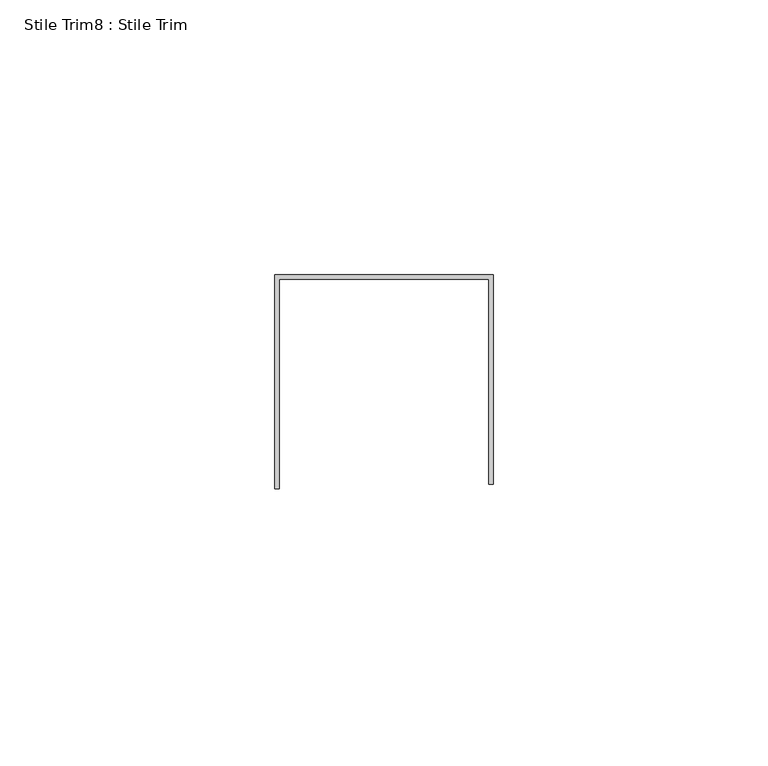
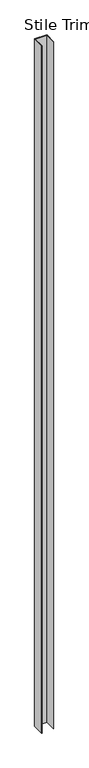
"""IFC4 building model written with IfcOpenShell, lengths in millimetres: proxy geometry, Stile Trim8 : Stile Trim."""

import ifcopenshell
import ifcopenshell.guid

model = None  # the IFC model being written
_history = None  # IfcOwnerHistory: only IFC2X3 demands one
_inside = {}  # id of a spatial element -> (the spatial element, [elements in it])
_under = {}  # id of a project, library or spatial element -> (it, [spatial elements below it])
_declared = {}  # id of a project -> (the project, [libraries it declares])
_typed = {}  # id of a type object -> (the type object, [elements of that type])
_made_of = {}  # id of a material, layer set ... -> (it, [elements and type objects made of it])


def new_model(schema):
    """Start an empty IFC model of exactly this schema.

    Asked for "IFC4X3", IfcOpenShell would pick the latest addendum, in which some entities
    have other attributes; the version numbers below select the first issue.
    IFC2X3 requires an IfcOwnerHistory on every rooted entity: one is made here for all.
    """
    global model, _history
    if schema == "IFC4X3":
        model = ifcopenshell.file(schema_version=(4, 3, 0, 0))
    else:
        model = ifcopenshell.file(schema=schema)
    _inside.clear()
    _under.clear()
    _declared.clear()
    _typed.clear()
    _made_of.clear()
    _history = None
    if model.schema == "IFC2X3":
        org = make("IfcOrganization", Name="unknown")
        user = make(
            "IfcPersonAndOrganization",
            ThePerson=make("IfcPerson", FamilyName="unknown"),
            TheOrganization=org,
        )
        app = make(
            "IfcApplication",
            ApplicationDeveloper=org,
            Version="unknown",
            ApplicationFullName="unknown",
            ApplicationIdentifier="unknown",
        )
        _history = make(
            "IfcOwnerHistory",
            OwningUser=user,
            OwningApplication=app,
            ChangeAction="ADDED",
            CreationDate=0,
        )
    return model


def make(cls, **values):
    """One entity of the class cls with the attributes given. An attribute that is None is left unset."""
    return model.create_entity(
        cls, **{name: value for name, value in values.items() if value is not None}
    )


def rooted(cls, **values):
    """An entity with a GlobalId (a new one), such as an element, a storey or a relation."""
    return make(cls, GlobalId=ifcopenshell.guid.new(), OwnerHistory=_history, **values)


def si_unit(unit_type, name, prefix=None):
    """IfcSIUnit, for example si_unit("LENGTHUNIT", "METRE", prefix="MILLI")."""
    return make("IfcSIUnit", UnitType=unit_type, Prefix=prefix, Name=name)


def assignment(units):
    """IfcUnitAssignment: the units of a project."""
    return None if units is None else make("IfcUnitAssignment", Units=units)


def point(xyz):
    """IfcCartesianPoint."""
    return None if xyz is None else make("IfcCartesianPoint", Coordinates=xyz)


def direction(xyz):
    """IfcDirection."""
    return None if xyz is None else make("IfcDirection", DirectionRatios=xyz)


def frame(location, z_axis=None, x_axis=None):
    """IfcAxis2Placement3D, a coordinate frame: its origin and axes. An axis left out is left unset."""
    return make(
        "IfcAxis2Placement3D",
        Location=point(location),
        Axis=direction(z_axis),
        RefDirection=direction(x_axis),
    )


def origin():
    """The frame at (0, 0, 0) with its axes left unset."""
    return frame((0.0, 0.0, 0.0))


def place(relative_to, where):
    """IfcLocalPlacement: puts the frame where relative to a parent placement (None: the world)."""
    return make(
        "IfcLocalPlacement", PlacementRelTo=relative_to, RelativePlacement=where
    )


def context(
    kind, dimensions, precision=None, world=None, true_north=None, identifier=None
):
    """IfcGeometricRepresentationContext, for example the 3D "Model" context."""
    return make(
        "IfcGeometricRepresentationContext",
        ContextIdentifier=identifier,
        ContextType=kind,
        CoordinateSpaceDimension=dimensions,
        Precision=precision,
        WorldCoordinateSystem=world,
        TrueNorth=true_north,
    )


def project(units=None, contexts=None):
    """IfcProject with its units and contexts."""
    return rooted(
        "IfcProject",
        Name="project",
        RepresentationContexts=contexts,
        UnitsInContext=assignment(units),
    )


def spatial(cls, under=None, at=None, **own):
    """A site, building, storey or space (cls), placed at a placement, below another one or the project."""
    s = rooted(cls, ObjectPlacement=at, **own)
    if under is not None:
        _under.setdefault(under.id(), (under, []))[1].append(s)
    return s


def polyline(points):
    """IfcPolyline through the points."""
    return make("IfcPolyline", Points=[point(p) for p in points])


def outline(outer, holes=None, kind="AREA"):
    """IfcArbitraryClosedProfileDef: a profile drawn as a closed curve; with holes, ...WithVoids."""
    if holes is None:
        return make("IfcArbitraryClosedProfileDef", ProfileType=kind, OuterCurve=outer)
    return make(
        "IfcArbitraryProfileDefWithVoids",
        ProfileType=kind,
        OuterCurve=outer,
        InnerCurves=holes,
    )


def extrude(swept, where, along, depth):
    """IfcExtrudedAreaSolid: the profile swept, set in the frame where, extruded along a direction by depth."""
    return make(
        "IfcExtrudedAreaSolid",
        SweptArea=swept,
        Position=where,
        ExtrudedDirection=direction(along),
        Depth=depth,
    )


def shape(context_of_items, identifier, shape_type, items):
    """IfcShapeRepresentation: the items that make up one representation, for example the "Body"."""
    return make(
        "IfcShapeRepresentation",
        ContextOfItems=context_of_items,
        RepresentationIdentifier=identifier,
        RepresentationType=shape_type,
        Items=items,
    )


def source(mapping_origin, context_of_items, identifier, shape_type, items):
    """IfcRepresentationMap: a shape defined once, which mapped items show again and again."""
    return make(
        "IfcRepresentationMap",
        MappingOrigin=mapping_origin,
        MappedRepresentation=shape(context_of_items, identifier, shape_type, items),
    )


def transform(
    local_origin,
    x_axis=None,
    y_axis=None,
    z_axis=None,
    scale=None,
    scale2=None,
    scale3=None,
    uniform=True,
):
    """IfcCartesianTransformationOperator3D, or its non-uniform kind. x_axis, y_axis, z_axis: its Axis1, 2, 3."""
    if uniform:
        return make(
            "IfcCartesianTransformationOperator3D",
            Axis1=direction(x_axis),
            Axis2=direction(y_axis),
            LocalOrigin=point(local_origin),
            Scale=scale,
            Axis3=direction(z_axis),
        )
    return make(
        "IfcCartesianTransformationOperator3DnonUniform",
        Axis1=direction(x_axis),
        Axis2=direction(y_axis),
        LocalOrigin=point(local_origin),
        Scale=scale,
        Axis3=direction(z_axis),
        Scale2=scale2,
        Scale3=scale3,
    )


def mapped(mapping_source, mapping_target):
    """IfcMappedItem: shows the shape of a source again, moved by a transform."""
    return make(
        "IfcMappedItem", MappingSource=mapping_source, MappingTarget=mapping_target
    )


def made_of(thing, what):
    """Note that an element or type object is made of a material, layer set ...; save() writes the relation."""
    if what is not None:
        _made_of.setdefault(what.id(), (what, []))[1].append(thing)
    return thing


def element(
    cls,
    number,
    at=None,
    inside=None,
    cuts=None,
    type_object=None,
    material=None,
    context=None,
    identifier="Body",
    shape_type=None,
    held_by="IfcProductDefinitionShape",
    body=None,
    shapes=None,
    **own,
):
    """One element of the class cls, such as IfcWall. Its Tag is "e" and its number.

    at: its placement. inside: the storey or other place that contains it. cuts: it is an
    opening in that element (IfcRelVoidsElement). A single representation is given by context,
    identifier, shape_type and body (its items); several are given by shapes. held_by: the class
    of the entity that holds the representations. save() writes the other relations.
    """
    e = rooted(cls, Tag="e%d" % number, ObjectPlacement=at, **own)
    if body is not None:
        shapes = [shape(context, identifier, shape_type, body)]
    if shapes is not None:
        e.Representation = make(held_by, Representations=shapes)
    if inside is not None:
        _inside.setdefault(inside.id(), (inside, []))[1].append(e)
    if cuts is not None:
        rooted(
            "IfcRelVoidsElement", RelatingBuildingElement=cuts, RelatedOpeningElement=e
        )
    if type_object is not None:
        _typed.setdefault(type_object.id(), (type_object, []))[1].append(e)
    return made_of(e, material)


def aggregate(whole, parts):
    """IfcRelAggregates: a whole, such as a stair, and the parts it consists of."""
    return rooted("IfcRelAggregates", RelatingObject=whole, RelatedObjects=parts)


def save(model, path):
    """Write the relations noted so far, then the file.

    IfcRelAggregates (storeys below a building ...), IfcRelContainedInSpatialStructure (elements
    in a storey), IfcRelDefinesByType, IfcRelAssociatesMaterial and IfcRelDeclares: one each for
    every whole, place, type object, material and project.
    """
    for whole, parts in _under.values():
        aggregate(whole, parts)
    for where, things in _inside.values():
        rooted(
            "IfcRelContainedInSpatialStructure",
            RelatedElements=things,
            RelatingStructure=where,
        )
    for kind, things in _typed.values():
        rooted("IfcRelDefinesByType", RelatedObjects=things, RelatingType=kind)
    for what, things in _made_of.values():
        rooted("IfcRelAssociatesMaterial", RelatedObjects=things, RelatingMaterial=what)
    for by, libraries in _declared.values():
        rooted("IfcRelDeclares", RelatingContext=by, RelatedDefinitions=libraries)
    model.write(path)


def stile_trim8_stile_trim_18cce888(model_context):
    return source(origin(), model_context, "Body", "SweptSolid", [
        extrude(outline(polyline([(587327.0060739, -535207.1289841), (587366.6808739, -535207.1289841), (587366.6808739, -535245.2289841), (587365.8934739, -535245.2289841), (587365.8934739, -535207.9163841), (587327.7934739, -535207.9163841), (587327.7934739, -535246.0163841), (587327.0060739, -535246.0163841), (587327.0060739, -535207.1289841)])), frame((0.0, 0.0, 50.8), z_axis=(0.0, 0.0, 1.0), x_axis=(1.0, 0.0, 0.0)), (0.0, 0.0, 1.0), 2350.3929688),
    ])


if __name__ == "__main__":
    model = new_model("IFC4")
    model_context = context("Model", 3, world=origin())
    ifc_project = project(units=[si_unit("LENGTHUNIT", "METRE", prefix="MILLI")], contexts=[model_context])
    site = spatial("IfcSite", under=ifc_project)
    building = spatial("IfcBuilding", under=site)
    placement = place(None, origin())
    stile_trim8_stile_trim_shape = stile_trim8_stile_trim_18cce888(model_context)
    element("IfcBuildingElementProxy", 1, Name="Stile Trim8 : Stile Trim", ObjectType="Stile Trim8 : Stile Trim", at=placement, inside=building, context=model_context, shape_type="MappedRepresentation", body=[
        mapped(stile_trim8_stile_trim_shape, transform((0.0, 0.0, 0.0), x_axis=(1.0, 0.0, 0.0), y_axis=(0.0, 1.0, 0.0), z_axis=(0.0, 0.0, 1.0))),
    ])
    save(model, "model.ifc")

# Revit data of these elements
# Element 1 (IfcBuildingElementProxy, "Stile Trim8 : Stile Trim")
#   Materials on its faces: "EDGE TRIM BY MTL PANEL MFR."
# Materials
#   "EDGE TRIM BY MTL PANEL MFR.": class "Generic", colour RGB 239 242 240, transparency 0, Cost = 0
